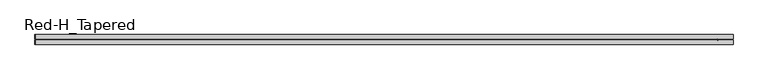
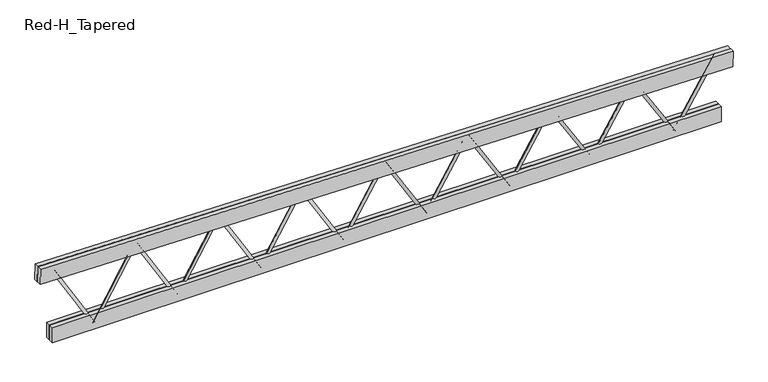
"""IFC4 building model written with IfcOpenShell, lengths in millimetres: beam geometry, Construction_Frames_RedBuilt_Openweb_Red-H_Tapered : Red-H_Tapered."""

from ifc_helpers import new_model, si_unit, point, frame, origin, origin_2d, place, context, project, spatial, polyline, circle_curve, trimmed, segment, composite_curve, outline, extrude, source, transform, mapped, element, save


def red_h_tapered_ce24421a(model_context):
    return source(origin(), model_context, "Body", "SweptSolid", [
        extrude(outline(composite_curve([segment(trimmed(circle_curve(origin_2d(), 12.7), [point((0.0, 12.7))], [point((0.0, -12.7))], False, "CARTESIAN"), True, "CONTINUOUS"), segment(trimmed(circle_curve(origin_2d(), 12.7), [point((0.0, -12.7))], [point((0.0, 12.7))], False, "CARTESIAN"), True, "CONTINUOUS")], self_intersect=False)), frame((2515.0014939, 0.0, -367.0101562), z_axis=(0.5238628746877267, 0.0, 0.8518026112450648), x_axis=(0.0, -1.0, 0.0)), (0.0, 0.0, 1.0), 685.8396444),
        extrude(outline(composite_curve([segment(trimmed(circle_curve(origin_2d(), 12.7), [point((0.0, -12.7000001))], [point((0.0, 12.7))], False, "CARTESIAN"), True, "CONTINUOUS"), segment(trimmed(circle_curve(origin_2d(), 12.7), [point((0.0, 12.7))], [point((0.0, -12.7000001))], False, "CARTESIAN"), True, "CONTINUOUS")], self_intersect=False)), frame((2515.0014939, 0.0, -367.0101562), z_axis=(-0.5212917882884671, 0.0, 0.8533785042189731), x_axis=(0.0, -1.0, 0.0)), (0.0, 0.0, 1.0), 689.2223046),
        extrude(outline(composite_curve([segment(trimmed(circle_curve(origin_2d(), 12.7), [point((0.0, 12.7))], [point((0.0, -12.7))], False, "CARTESIAN"), True, "CONTINUOUS"), segment(trimmed(circle_curve(origin_2d(), 12.7), [point((0.0, -12.7))], [point((0.0, 12.7))], False, "CARTESIAN"), True, "CONTINUOUS")], self_intersect=False)), frame((1796.4296385, 0.0, -367.0101562), z_axis=(0.5212917882884663, 0.0, 0.8533785042189738), x_axis=(0.0, -1.0, 0.0)), (0.0, 0.0, 1.0), 689.2223046),
        extrude(outline(composite_curve([segment(trimmed(circle_curve(origin_2d(), 12.7), [point((0.0, -12.7000001))], [point((0.0, 12.6999999))], False, "CARTESIAN"), True, "CONTINUOUS"), segment(trimmed(circle_curve(origin_2d(), 12.7), [point((0.0, 12.6999999))], [point((0.0, -12.7000001))], False, "CARTESIAN"), True, "CONTINUOUS")], self_intersect=False)), frame((1796.4296385, 0.0, -367.0101562), z_axis=(-0.5187411676162864, 0.0, 0.8549313428691757), x_axis=(0.0, -1.0, 0.0)), (0.0, 0.0, 1.0), 692.6111713),
        extrude(outline(composite_curve([segment(trimmed(circle_curve(origin_2d(), 12.7), [point((0.0, 12.7))], [point((0.0, -12.7))], False, "CARTESIAN"), True, "CONTINUOUS"), segment(trimmed(circle_curve(origin_2d(), 12.7), [point((0.0, -12.7))], [point((0.0, 12.7))], False, "CARTESIAN"), True, "CONTINUOUS")], self_intersect=False)), frame((1077.8577831, 0.0, -367.0101562), z_axis=(0.5187411676162853, 0.0, 0.8549313428691763), x_axis=(0.0, -1.0, 0.0)), (0.0, 0.0, 1.0), 692.6111713),
        extrude(outline(composite_curve([segment(trimmed(circle_curve(origin_2d(), 12.7), [point((0.0, -12.7))], [point((0.0, 12.7))], False, "CARTESIAN"), True, "CONTINUOUS"), segment(trimmed(circle_curve(origin_2d(), 12.7), [point((0.0, 12.7))], [point((0.0, -12.7))], False, "CARTESIAN"), True, "CONTINUOUS")], self_intersect=False)), frame((1077.8577831, 0.0, -367.0101562), z_axis=(-0.5162108492002061, 0.0, 0.8564615339686903), x_axis=(0.0, -1.0, 0.0)), (0.0, 0.0, 1.0), 696.0061538),
        extrude(outline(composite_curve([segment(trimmed(circle_curve(origin_2d(), 12.7), [point((0.0, 12.7))], [point((0.0, -12.7))], False, "CARTESIAN"), True, "CONTINUOUS"), segment(trimmed(circle_curve(origin_2d(), 12.7), [point((0.0, -12.7))], [point((0.0, 12.7))], False, "CARTESIAN"), True, "CONTINUOUS")], self_intersect=False)), frame((359.2859277, 0.0, -367.0101562), z_axis=(0.5162108492002068, 0.0, 0.85646153396869), x_axis=(0.0, -1.0, 0.0)), (0.0, 0.0, 1.0), 696.0061538),
        extrude(outline(composite_curve([segment(trimmed(circle_curve(origin_2d(), 12.7), [point((0.0, -12.7))], [point((0.0, 12.6999999))], False, "CARTESIAN"), True, "CONTINUOUS"), segment(trimmed(circle_curve(origin_2d(), 12.7), [point((0.0, 12.6999999))], [point((0.0, -12.7))], False, "CARTESIAN"), True, "CONTINUOUS")], self_intersect=False)), frame((359.2859277, 0.0, -367.0101562), z_axis=(-0.5137006691841376, 0.0, 0.8579694764266206), x_axis=(0.0, -1.0, 0.0)), (0.0, 0.0, 1.0), 699.4071631),
        extrude(outline(composite_curve([segment(trimmed(circle_curve(origin_2d(), 12.7), [point((0.0, -12.6999999))], [point((0.0, 12.7))], False, "CARTESIAN"), True, "CONTINUOUS"), segment(trimmed(circle_curve(origin_2d(), 12.7), [point((0.0, 12.7))], [point((0.0, -12.6999999))], False, "CARTESIAN"), True, "CONTINUOUS")], self_intersect=False)), frame((-359.2859277, 0.0, -367.0101562), z_axis=(0.5137006691841062, 0.0, 0.8579694764266393), x_axis=(0.0, -1.0, 0.0)), (0.0, 0.0, 1.0), 699.4071631),
        extrude(outline(composite_curve([segment(trimmed(circle_curve(origin_2d(), 12.7), [point((0.0, 12.6999999))], [point((0.0, -12.7))], False, "CARTESIAN"), True, "CONTINUOUS"), segment(trimmed(circle_curve(origin_2d(), 12.7), [point((0.0, -12.7))], [point((0.0, 12.6999999))], False, "CARTESIAN"), True, "CONTINUOUS")], self_intersect=False)), frame((-359.2859277, 0.0, -367.0101562), z_axis=(-0.5112104634271233, 0.0, 0.8594555614356254), x_axis=(0.0, -1.0, 0.0)), (0.0, 0.0, 1.0), 702.8141116),
        extrude(outline(composite_curve([segment(trimmed(circle_curve(origin_2d(), 12.7), [point((0.0, -12.6999999))], [point((0.0, 12.7000001))], False, "CARTESIAN"), True, "CONTINUOUS"), segment(trimmed(circle_curve(origin_2d(), 12.7), [point((0.0, 12.7000001))], [point((0.0, -12.6999999))], False, "CARTESIAN"), True, "CONTINUOUS")], self_intersect=False)), frame((-1077.8577831, 0.0, -367.0101562), z_axis=(0.5112104634271216, 0.0, 0.8594555614356263), x_axis=(0.0, -1.0, 0.0)), (0.0, 0.0, 1.0), 702.8141116),
        extrude(outline(composite_curve([segment(trimmed(circle_curve(origin_2d(), 12.7), [point((0.0, 12.7))], [point((0.0, -12.7))], False, "CARTESIAN"), True, "CONTINUOUS"), segment(trimmed(circle_curve(origin_2d(), 12.7), [point((0.0, -12.7))], [point((0.0, 12.7))], False, "CARTESIAN"), True, "CONTINUOUS")], self_intersect=False)), frame((-1077.8577831, 0.0, -367.0101562), z_axis=(-0.5087400675988173, 0.0, 0.8609201726173867), x_axis=(0.0, -1.0, 0.0)), (0.0, 0.0, 1.0), 706.2269135),
        extrude(outline(composite_curve([segment(trimmed(circle_curve(origin_2d(), 12.7), [point((0.0, -12.7))], [point((0.0, 12.7))], False, "CARTESIAN"), True, "CONTINUOUS"), segment(trimmed(circle_curve(origin_2d(), 12.7), [point((0.0, 12.7))], [point((0.0, -12.7))], False, "CARTESIAN"), True, "CONTINUOUS")], self_intersect=False)), frame((-1796.4296385, 0.0, -367.0101562), z_axis=(0.5087400675988304, 0.0, 0.8609201726173789), x_axis=(0.0, -1.0, 0.0)), (0.0, 0.0, 1.0), 706.2269135),
        extrude(outline(composite_curve([segment(trimmed(circle_curve(origin_2d(), 12.7), [point((0.0, 12.7))], [point((0.0, -12.7))], False, "CARTESIAN"), True, "CONTINUOUS"), segment(trimmed(circle_curve(origin_2d(), 12.7), [point((0.0, -12.7))], [point((0.0, 12.7))], False, "CARTESIAN"), True, "CONTINUOUS")], self_intersect=False)), frame((-1796.4296385, 0.0, -367.0101562), z_axis=(-0.5062893172698286, 0.0, 0.8623636861663707), x_axis=(0.0, -1.0, 0.0)), (0.0, 0.0, 1.0), 709.6454842),
        extrude(outline(composite_curve([segment(trimmed(circle_curve(origin_2d(), 12.7), [point((0.0, -12.7))], [point((0.0, 12.7000001))], False, "CARTESIAN"), True, "CONTINUOUS"), segment(trimmed(circle_curve(origin_2d(), 12.7), [point((0.0, 12.7000001))], [point((0.0, -12.7))], False, "CARTESIAN"), True, "CONTINUOUS")], self_intersect=False)), frame((-2515.0014939, 0.0, -367.0101562), z_axis=(0.506289317269817, 0.0, 0.8623636861663776), x_axis=(0.0, -1.0, 0.0)), (0.0, 0.0, 1.0), 709.6454842),
        extrude(outline(composite_curve([segment(trimmed(circle_curve(origin_2d(), 12.7), [point((0.0, 12.7))], [point((0.0, -12.7))], False, "CARTESIAN"), True, "CONTINUOUS"), segment(trimmed(circle_curve(origin_2d(), 12.7), [point((0.0, -12.7))], [point((0.0, 12.7))], False, "CARTESIAN"), True, "CONTINUOUS")], self_intersect=False)), frame((-2515.0014939, 0.0, -367.0101562), z_axis=(-0.5038580479976417, 0.0, 0.8637864709915329), x_axis=(0.0, -1.0, 0.0)), (0.0, 0.0, 1.0), 713.0697408),
        extrude(outline(polyline([(-2899.6874215, -41.275), (-2899.6874215, -3.175), (2899.6874215, -3.175), (2899.6874215, -41.275), (-2899.6874215, -41.275)])), frame((0.0, 0.0, -386.0601562), z_axis=(0.0, 0.0, 1.0), x_axis=(1.0, 0.0, 0.0)), (0.0, 0.0, 1.0), 139.7),
        extrude(outline(polyline([(-2899.6874215, 3.175), (-2899.6874215, 41.275), (2899.6874215, 41.275), (2899.6874215, 3.175), (-2899.6874215, 3.175)])), frame((0.0, 0.0, -386.0601562), z_axis=(0.0, 0.0, 1.0), x_axis=(1.0, 0.0, 0.0)), (0.0, 0.0, 1.0), 139.7),
        extrude(outline(polyline([(0.0, -38.1), (0.0, 0.0), (6003.4346259, 0.0), (6003.4346259, -38.1), (0.0, -38.1)])), frame((-3003.6516548, -3.175, 185.4598509), z_axis=(0.01692364560154548, 0.0, 0.9998567848544877), x_axis=(0.9998567848544877, 0.0, -0.01692364560154548)), (0.0, 0.0, 1.0), 139.7),
        extrude(outline(polyline([(0.0, -38.1), (0.0, 0.0), (6003.4346259, 0.0), (6003.4346259, -38.1), (0.0, -38.1)])), frame((-3003.6516548, 41.275, 185.4598509), z_axis=(0.01692364560154548, 0.0, 0.9998567848544877), x_axis=(0.9998567848544877, 0.0, -0.01692364560154548)), (0.0, 0.0, 1.0), 139.7),
    ])


if __name__ == "__main__":
    model = new_model("IFC4")
    model_context = context("Model", 3, world=origin())
    ifc_project = project(units=[si_unit("LENGTHUNIT", "METRE", prefix="MILLI")], contexts=[model_context])
    site = spatial("IfcSite", under=ifc_project)
    building = spatial("IfcBuilding", under=site)
    placement = place(None, origin())
    red_h_tapered_shape = red_h_tapered_ce24421a(model_context)
    element("IfcBeam", 1, ObjectType="Construction_Frames_RedBuilt_Openweb_Red-H_Tapered : Red-H_Tapered", at=placement, inside=building, context=model_context, shape_type="MappedRepresentation", body=[
        mapped(red_h_tapered_shape, transform((0.0, 0.0, 0.0), x_axis=(1.0, 0.0, 0.0), y_axis=(0.0, 1.0, 0.0), z_axis=(0.0, 0.0, 1.0))),
    ])
    save(model, "model.ifc")

# Revit data of these elements
# Type "Construction_Frames_RedBuilt_Openweb_Red-H_Tapered : Red-H_Tapered"
#   Youtube clip = ""
#   Weight Net (Kg) = "0"
#   Webs = "Up to 2\" diameter tubular steel"
#   Uniformat II Description = ""
#   Uniformat II Code = ""
#   Uniclass 2015 Name = "Softwood trusses"
#   Uniclass 2015 Code = "Pr_20_85_90_81"
#   Uniclass 2.0 Description = "Structural Framing Systems"
#   Uniclass 2.0 Code = "SS-15-10-75"
#   Uniclass 1.4 Description = "Trusses"
#   Uniclass 1.4 Code = "L3523"
#   UNSPSC Code = "30103606"
#   Technical description = "http://www.redbuilt.com/reference/literature-and-other-resources"
#   Region South America = "None"
#   Region Oceania = "None"
#   Region North America = "US"
#   Region Middle East = "None"
#   Region Europe = "None"
#   Region Asia = "None"
#   Region Antarctica = "None"
#   Region Africa = "None"
#   QR code = "http://bimobject.com/redbuilt/product/redbuilt-0003"
#   Product url = "http://www.redbuilt.com/products/default.aspx?id=2"
#   Product group = "Wood Trusses"
#   Product family = "Construction"
#   Product data url = "https://bimobject.com/redbuilt/product/redbuilt-0003"
#   Product certification = ""
#   Product SKU = "redbuilt-0003"
#   Product Page URL = "http://www.redbuilt.com/commercial-systems/red-m-red-h-open-web-trusses"
#   Product Guid = "2c5793f2-6ffb-4665-b825-cf90c048e711"
#   Product Documentation Link = "http://www.redbuilt.com/documents/OW_Guide_2017_07_LowRes_wLinks.pdf"
#   OmniClass Description = "Wood Trusses"
#   OmniClass Code = "23-13 35 19 13 17"
#   NBS Reference Description = ""
#   NBS Reference Code = ""
#   Material secondary = "Steel"
#   Material main = "CHARRED WOOD"
#   Masterformat 2014 Description = "Metal-Web Wood Joists"
#   Masterformat 2014 Code = "06 17 36"
#   Manufacturer name = "RedBuilt"
#   Manufacturer country = "United States"
#   Installation instructions = "http://www.redbuilt.com/documents/Installation_Sheets_Open-Web.pdf"
#   IFC Classification = ""
#   EAN code = ""
#   Design country = "United States"
#   Product Information = "http://redbuilt.com/products/default.aspx?id=2"
#   Model = "Red-H-Tapered"
#   Manufacturer URL = "http://redbuilt.com/"
#   Manufacturer = "RedBuilt™"
#   Description = "Open Web Truss"
#   Date of publishing = "8/17/2010"
#   Contact us = "http://redbuilt.com/contact/"
#   Chords = "Double 1½\" x 5½\" MSR lumber"
#   COBIe Type Category = ""
#   Brand url = "http://www.redbuilt.com"
#   BIMobject main category code = "construction"
#   BIMobject main category = "Construction"
#   BIMobject category code = "construction-frames-trusses"
#   BIMobject category = "Frames & Trusses"
#   Web Radius = 0' - 0 1/2"
#   Web Layout Offset Start [instance default] = 0' - 5"
#   Web Layout Offset End [instance default] = 0' - 5"
#   Web Diameter = 0' - 1"
#   TotalLength [instance default] = 20' - 0"
#   Span Minimum = 4' - 0"
#   Span Maximum = 70' - 0"
#   Span Limit [instance default] = 20' - 0"
#   Nominal width = 0' - 0"
#   Nominal height = 0' - 0"
#   Inner Depth Top [instance default] = 0' - 2.76372"
#   Depth Start [instance default] = 6' - 0"
#   Top Chord Length [instance default] = 20' - 1.19701"
#   TC Extension Start Aux [instance default] = 0' - 0"
#   TC Extension End Aux [instance default] = 0' - 0"
#   T-B Chord Length Difference L [instance default] = 0' - 4"
#   T-B Chord Length Difference [instance default] = 0' - 4"
#   Height 2 [instance default] = 6' - 0"
#   Depth Minimum at Wall = 2' - 0"
#   Depth Maximum at Wall = 6' - 0"
#   Depth Lower End [instance default] = 2' - 0"
#   Depth Higher End [instance default] = 6' - 0"
#   Depth End [instance default] = 2' - 0"
#   Depth 2 [instance default] = 2' - 0"
#   Chord Width = 0' - 3 1/4"
#   Chord Thickness = 0' - 1 1/2"
#   Chord Depth = 0' - 5 1/2"
#   Offset Start [instance default] = 0' - 0"
#   TC Extension Start [instance default] = 0' - 0"
#   End Panel = 0' - 5"
#   Offset End [instance default] = 0' - 0"
#   TC Extension End [instance default] = 0' - 0"
#   Length [instance default] = 20' - 0"
#   Angle [instance default] = 5.71059°
#   Span Limit Warning [instance default] = no
#   Edition number = 1
#   Top Bearing Start [instance default] = yes
#   Top Bearing End [instance default] = yes
#   Bottom Bearing Start [instance default] = no
#   Bottom Bearing End [instance default] = no
#   8 Panels [instance default] = yes
#   16 Panels [instance default] = no
#   12 Panels [instance default] = no
#   Web Material = RedBuilt-Steel, Galvanized
#   Clip Material = RedBuilt-Steel, Galvanized
#   Chords Material = WOOD-OAKFIRE
#   URL = ""
#   Assembly Code = ""
# Element 1 (IfcBeam, "Construction_Frames_RedBuilt_Openweb_Red-H_Tapered : Red-H_Tapered")
#   TotalLength = 19' - 8.32184"
#   Span Limit = 19' - 8.32184"
#   Inner Depth Top = 0' - 2.75039"
#   Depth Start = 5' - 0"
#   Top Chord Length = 19' - 8.35569"
#   Height 2 = 5' - 0"
#   Depth Higher End = 5' - 0"
#   Depth 2 = 0' - 4"
#   Angle = 0.9697°
#   Materials on its faces: "RedBuilt-Steel, Galvanized", "WOOD-OAKFIRE"
# Materials
#   "RedBuilt-Steel, Galvanized": class "Metal", colour RGB 164 172 176, transparency 0, Manufacturer = "RedBuilt. LLC", Comments = "Openweb Metal Web", URL = "http://www.redbuilt.com/", Description = "Galvanized steel", Cost = 0
#   "WOOD-OAKFIRE": class "Wood", colour RGB 198 202 183, transparency 0, Description = "Generic wood", Cost = 0
